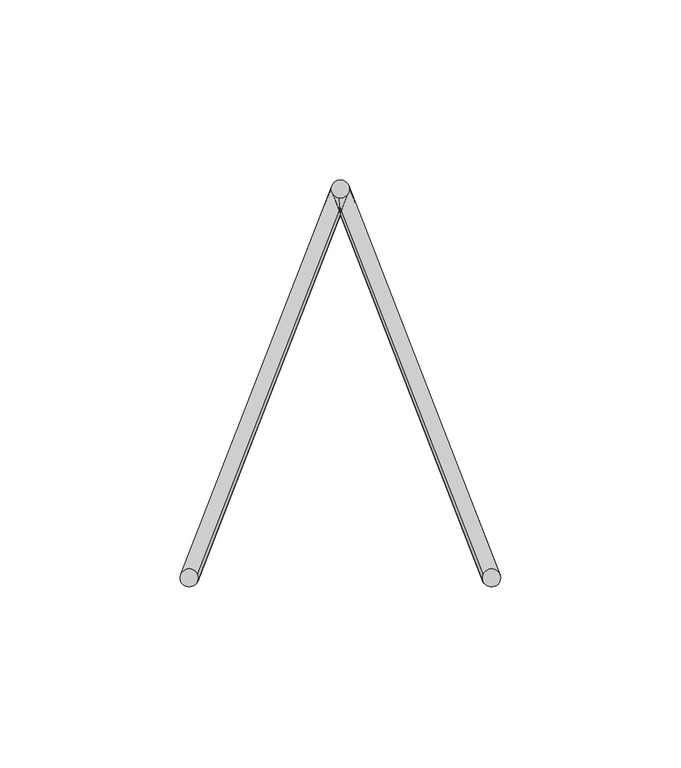
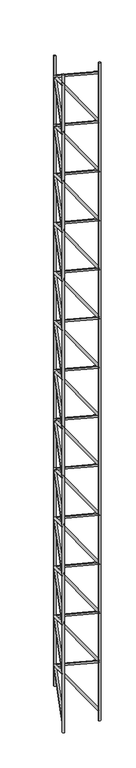
"""IFC4 building model written with IfcOpenShell, lengths in millimetres: proxy geometry, Pre-fab. (Vigota 2 - Pano 8)."""

from ifc_helpers import new_model, si_unit, point, frame, frame_2d, origin, origin_with_axes, origin_2d, place, context, project, spatial, circle_curve, trimmed, segment, composite_curve, outline, extrude, source, transform, mapped, element, save


def structural_framing_c6495f8e(model_context):
    return source(origin(), model_context, "Body", "SweptSolid", [
        extrude(outline(composite_curve([segment(trimmed(circle_curve(origin_2d(), 2.5), [point((2.5, 0.0))], [point((-2.5, 0.0))], False, "CARTESIAN"), True, "CONTINUOUS"), segment(trimmed(circle_curve(origin_2d(), 2.5), [point((-2.5, 0.0))], [point((2.5, 0.0))], False, "CARTESIAN"), True, "CONTINUOUS")], self_intersect=False)), origin_with_axes(), (0.0, 0.0, 1.0), 1607.655183),
        extrude(outline(composite_curve([segment(trimmed(circle_curve(frame_2d((-42.0, 108.0)), 2.5), [point((-39.5, 108.0))], [point((-44.5, 108.0))], False, "CARTESIAN"), True, "CONTINUOUS"), segment(trimmed(circle_curve(frame_2d((-42.0, 108.0)), 2.5), [point((-44.5, 108.0))], [point((-39.5, 108.0))], False, "CARTESIAN"), True, "CONTINUOUS")], self_intersect=False)), frame((0.0, 0.0, 33.8275917), z_axis=(0.0, 0.0, 1.0), x_axis=(1.0, 0.0, 0.0)), (0.0, 0.0, 1.0), 1540.0),
        extrude(outline(composite_curve([segment(trimmed(circle_curve(origin_2d(), 2.5), [point((2.5, 0.0))], [point((-2.5, 0.0))], False, "CARTESIAN"), True, "CONTINUOUS"), segment(trimmed(circle_curve(origin_2d(), 2.5), [point((-2.5, 0.0))], [point((2.5, 0.0))], False, "CARTESIAN"), True, "CONTINUOUS")], self_intersect=False)), frame((0.0, 0.0, 23.8275917), z_axis=(-0.3218603428886276, 0.8276408817707567, 0.4598004898837537), x_axis=(0.8192319205108605, -3.936835275445103e-11, 0.5734623443750141)), (0.0, 0.0, 1.0), 130.491379),
        extrude(outline(composite_curve([segment(trimmed(circle_curve(origin_2d(), 2.5), [point((2.5, 0.0))], [point((-2.5, 0.0))], False, "CARTESIAN"), True, "CONTINUOUS"), segment(trimmed(circle_curve(origin_2d(), 2.5), [point((-2.5, 0.0))], [point((2.5, 0.0))], False, "CARTESIAN"), True, "CONTINUOUS")], self_intersect=False)), frame((-42.0, 108.0, 83.8275917), z_axis=(0.3218603428886276, -0.8276408817707567, 0.4598004898837537), x_axis=(0.8192319205108605, -3.936835275445103e-11, -0.5734623443750141)), (0.0, 0.0, 1.0), 130.491379),
        extrude(outline(composite_curve([segment(trimmed(circle_curve(origin_2d(), 2.5), [point((2.5, 0.0))], [point((-2.5, 0.0))], False, "CARTESIAN"), True, "CONTINUOUS"), segment(trimmed(circle_curve(origin_2d(), 2.5), [point((-2.5, 0.0))], [point((2.5, 0.0))], False, "CARTESIAN"), True, "CONTINUOUS")], self_intersect=False)), frame((0.0, 0.0, 143.8275917), z_axis=(-0.3218603428886276, 0.8276408817707567, 0.4598004898837537), x_axis=(0.8192319205108605, -3.936835275445103e-11, 0.5734623443750141)), (0.0, 0.0, 1.0), 130.491379),
        extrude(outline(composite_curve([segment(trimmed(circle_curve(origin_2d(), 2.5), [point((2.5, 0.0))], [point((-2.5, 0.0))], False, "CARTESIAN"), True, "CONTINUOUS"), segment(trimmed(circle_curve(origin_2d(), 2.5), [point((-2.5, 0.0))], [point((2.5, 0.0))], False, "CARTESIAN"), True, "CONTINUOUS")], self_intersect=False)), frame((-42.0, 108.0, 203.8275917), z_axis=(0.3218603428886276, -0.8276408817707567, 0.4598004898837537), x_axis=(0.8192319205108605, -3.936835275445103e-11, -0.5734623443750141)), (0.0, 0.0, 1.0), 130.491379),
        extrude(outline(composite_curve([segment(trimmed(circle_curve(origin_2d(), 2.5), [point((2.5, 0.0))], [point((-2.5, 0.0))], False, "CARTESIAN"), True, "CONTINUOUS"), segment(trimmed(circle_curve(origin_2d(), 2.5), [point((-2.5, 0.0))], [point((2.5, 0.0))], False, "CARTESIAN"), True, "CONTINUOUS")], self_intersect=False)), frame((0.0, 0.0, 263.8275917), z_axis=(-0.3218603428886276, 0.8276408817707567, 0.4598004898837537), x_axis=(0.8192319205108605, -3.936835275445103e-11, 0.5734623443750141)), (0.0, 0.0, 1.0), 130.491379),
        extrude(outline(composite_curve([segment(trimmed(circle_curve(origin_2d(), 2.5), [point((2.5, 0.0))], [point((-2.5, 0.0))], False, "CARTESIAN"), True, "CONTINUOUS"), segment(trimmed(circle_curve(origin_2d(), 2.5), [point((-2.5, 0.0))], [point((2.5, 0.0))], False, "CARTESIAN"), True, "CONTINUOUS")], self_intersect=False)), frame((-42.0, 108.0, 323.8275917), z_axis=(0.3218603428886276, -0.8276408817707567, 0.4598004898837537), x_axis=(0.8192319205108605, -3.936835275445103e-11, -0.5734623443750141)), (0.0, 0.0, 1.0), 130.491379),
        extrude(outline(composite_curve([segment(trimmed(circle_curve(origin_2d(), 2.5), [point((2.5, 0.0))], [point((-2.5, 0.0))], False, "CARTESIAN"), True, "CONTINUOUS"), segment(trimmed(circle_curve(origin_2d(), 2.5), [point((-2.5, 0.0))], [point((2.5, 0.0))], False, "CARTESIAN"), True, "CONTINUOUS")], self_intersect=False)), frame((0.0, 0.0, 383.8275917), z_axis=(-0.3218603428886276, 0.8276408817707567, 0.4598004898837537), x_axis=(0.8192319205108605, -3.936835275445103e-11, 0.5734623443750141)), (0.0, 0.0, 1.0), 130.491379),
        extrude(outline(composite_curve([segment(trimmed(circle_curve(origin_2d(), 2.5), [point((2.5, 0.0))], [point((-2.5, 0.0))], False, "CARTESIAN"), True, "CONTINUOUS"), segment(trimmed(circle_curve(origin_2d(), 2.5), [point((-2.5, 0.0))], [point((2.5, 0.0))], False, "CARTESIAN"), True, "CONTINUOUS")], self_intersect=False)), frame((-42.0, 108.0, 443.8275917), z_axis=(0.3218603428886276, -0.8276408817707567, 0.4598004898837537), x_axis=(0.8192319205108605, -3.936835275445103e-11, -0.5734623443750141)), (0.0, 0.0, 1.0), 130.491379),
        extrude(outline(composite_curve([segment(trimmed(circle_curve(origin_2d(), 2.5), [point((2.5, 0.0))], [point((-2.5, 0.0))], False, "CARTESIAN"), True, "CONTINUOUS"), segment(trimmed(circle_curve(origin_2d(), 2.5), [point((-2.5, 0.0))], [point((2.5, 0.0))], False, "CARTESIAN"), True, "CONTINUOUS")], self_intersect=False)), frame((0.0, 0.0, 503.8275917), z_axis=(-0.3218603428886276, 0.8276408817707567, 0.4598004898837537), x_axis=(0.8192319205108605, -3.936835275445103e-11, 0.5734623443750141)), (0.0, 0.0, 1.0), 130.491379),
        extrude(outline(composite_curve([segment(trimmed(circle_curve(origin_2d(), 2.5), [point((2.5, 0.0))], [point((-2.5, 0.0))], False, "CARTESIAN"), True, "CONTINUOUS"), segment(trimmed(circle_curve(origin_2d(), 2.5), [point((-2.5, 0.0))], [point((2.5, 0.0))], False, "CARTESIAN"), True, "CONTINUOUS")], self_intersect=False)), frame((-42.0, 108.0, 563.8275917), z_axis=(0.3218603428886276, -0.8276408817707567, 0.4598004898837537), x_axis=(0.8192319205108605, -3.936835275445103e-11, -0.5734623443750141)), (0.0, 0.0, 1.0), 130.491379),
        extrude(outline(composite_curve([segment(trimmed(circle_curve(origin_2d(), 2.5), [point((2.5, 0.0))], [point((-2.5, 0.0))], False, "CARTESIAN"), True, "CONTINUOUS"), segment(trimmed(circle_curve(origin_2d(), 2.5), [point((-2.5, 0.0))], [point((2.5, 0.0))], False, "CARTESIAN"), True, "CONTINUOUS")], self_intersect=False)), frame((0.0, 0.0, 623.8275917), z_axis=(-0.3218603428886276, 0.8276408817707567, 0.4598004898837537), x_axis=(0.8192319205108605, -3.936835275445103e-11, 0.5734623443750141)), (0.0, 0.0, 1.0), 130.491379),
        extrude(outline(composite_curve([segment(trimmed(circle_curve(origin_2d(), 2.5), [point((2.5, 0.0))], [point((-2.5, 0.0))], False, "CARTESIAN"), True, "CONTINUOUS"), segment(trimmed(circle_curve(origin_2d(), 2.5), [point((-2.5, 0.0))], [point((2.5, 0.0))], False, "CARTESIAN"), True, "CONTINUOUS")], self_intersect=False)), frame((-42.0, 108.0, 683.8275917), z_axis=(0.3218603428886276, -0.8276408817707567, 0.4598004898837537), x_axis=(0.8192319205108605, -3.936835275445103e-11, -0.5734623443750141)), (0.0, 0.0, 1.0), 130.491379),
        extrude(outline(composite_curve([segment(trimmed(circle_curve(origin_2d(), 2.5), [point((2.5, 0.0))], [point((-2.5, 0.0))], False, "CARTESIAN"), True, "CONTINUOUS"), segment(trimmed(circle_curve(origin_2d(), 2.5), [point((-2.5, 0.0))], [point((2.5, 0.0))], False, "CARTESIAN"), True, "CONTINUOUS")], self_intersect=False)), frame((0.0, 0.0, 743.8275917), z_axis=(-0.3218603428886276, 0.8276408817707567, 0.4598004898837537), x_axis=(0.8192319205108605, -3.936835275445103e-11, 0.5734623443750141)), (0.0, 0.0, 1.0), 130.491379),
        extrude(outline(composite_curve([segment(trimmed(circle_curve(origin_2d(), 2.5), [point((2.5, 0.0))], [point((-2.5, 0.0))], False, "CARTESIAN"), True, "CONTINUOUS"), segment(trimmed(circle_curve(origin_2d(), 2.5), [point((-2.5, 0.0))], [point((2.5, 0.0))], False, "CARTESIAN"), True, "CONTINUOUS")], self_intersect=False)), frame((-42.0, 108.0, 803.8275917), z_axis=(0.3218603428886276, -0.8276408817707567, 0.4598004898837537), x_axis=(0.8192319205108605, -3.936835275445103e-11, -0.5734623443750141)), (0.0, 0.0, 1.0), 130.491379),
        extrude(outline(composite_curve([segment(trimmed(circle_curve(origin_2d(), 2.5), [point((2.5, 0.0))], [point((-2.5, 0.0))], False, "CARTESIAN"), True, "CONTINUOUS"), segment(trimmed(circle_curve(origin_2d(), 2.5), [point((-2.5, 0.0))], [point((2.5, 0.0))], False, "CARTESIAN"), True, "CONTINUOUS")], self_intersect=False)), frame((0.0, 0.0, 863.8275917), z_axis=(-0.3218603428886276, 0.8276408817707567, 0.4598004898837537), x_axis=(0.8192319205108605, -3.936835275445103e-11, 0.5734623443750141)), (0.0, 0.0, 1.0), 130.491379),
        extrude(outline(composite_curve([segment(trimmed(circle_curve(origin_2d(), 2.5), [point((2.5, 0.0))], [point((-2.5, 0.0))], False, "CARTESIAN"), True, "CONTINUOUS"), segment(trimmed(circle_curve(origin_2d(), 2.5), [point((-2.5, 0.0))], [point((2.5, 0.0))], False, "CARTESIAN"), True, "CONTINUOUS")], self_intersect=False)), frame((-42.0, 108.0, 923.8275917), z_axis=(0.3218603428886276, -0.8276408817707567, 0.4598004898837537), x_axis=(0.8192319205108605, -3.936835275445103e-11, -0.5734623443750141)), (0.0, 0.0, 1.0), 130.491379),
        extrude(outline(composite_curve([segment(trimmed(circle_curve(origin_2d(), 2.5), [point((2.5, 0.0))], [point((-2.5, 0.0))], False, "CARTESIAN"), True, "CONTINUOUS"), segment(trimmed(circle_curve(origin_2d(), 2.5), [point((-2.5, 0.0))], [point((2.5, 0.0))], False, "CARTESIAN"), True, "CONTINUOUS")], self_intersect=False)), frame((0.0, 0.0, 983.8275917), z_axis=(-0.3218603428886276, 0.8276408817707567, 0.4598004898837537), x_axis=(0.8192319205108605, -3.936835275445103e-11, 0.5734623443750141)), (0.0, 0.0, 1.0), 130.491379),
        extrude(outline(composite_curve([segment(trimmed(circle_curve(origin_2d(), 2.5), [point((2.5, 0.0))], [point((-2.5, 0.0))], False, "CARTESIAN"), True, "CONTINUOUS"), segment(trimmed(circle_curve(origin_2d(), 2.5), [point((-2.5, 0.0))], [point((2.5, 0.0))], False, "CARTESIAN"), True, "CONTINUOUS")], self_intersect=False)), frame((-42.0, 108.0, 1043.827592), z_axis=(0.3218603428886276, -0.8276408817707567, 0.4598004898837537), x_axis=(0.8192319205108605, -3.936835275445103e-11, -0.5734623443750141)), (0.0, 0.0, 1.0), 130.491379),
        extrude(outline(composite_curve([segment(trimmed(circle_curve(origin_2d(), 2.5), [point((2.5, 0.0))], [point((-2.5, 0.0))], False, "CARTESIAN"), True, "CONTINUOUS"), segment(trimmed(circle_curve(origin_2d(), 2.5), [point((-2.5, 0.0))], [point((2.5, 0.0))], False, "CARTESIAN"), True, "CONTINUOUS")], self_intersect=False)), frame((0.0, 0.0, 1103.827592), z_axis=(-0.3218603428886276, 0.8276408817707567, 0.4598004898837537), x_axis=(0.8192319205108605, -3.936835275445103e-11, 0.5734623443750141)), (0.0, 0.0, 1.0), 130.491379),
        extrude(outline(composite_curve([segment(trimmed(circle_curve(origin_2d(), 2.5), [point((2.5, 0.0))], [point((-2.5, 0.0))], False, "CARTESIAN"), True, "CONTINUOUS"), segment(trimmed(circle_curve(origin_2d(), 2.5), [point((-2.5, 0.0))], [point((2.5, 0.0))], False, "CARTESIAN"), True, "CONTINUOUS")], self_intersect=False)), frame((-42.0, 108.0, 1163.827592), z_axis=(0.3218603428886276, -0.8276408817707567, 0.4598004898837537), x_axis=(0.8192319205108605, -3.936835275445103e-11, -0.5734623443750141)), (0.0, 0.0, 1.0), 130.491379),
        extrude(outline(composite_curve([segment(trimmed(circle_curve(origin_2d(), 2.5), [point((2.5, 0.0))], [point((-2.5, 0.0))], False, "CARTESIAN"), True, "CONTINUOUS"), segment(trimmed(circle_curve(origin_2d(), 2.5), [point((-2.5, 0.0))], [point((2.5, 0.0))], False, "CARTESIAN"), True, "CONTINUOUS")], self_intersect=False)), frame((0.0, 0.0, 1223.827592), z_axis=(-0.3218603428886276, 0.8276408817707567, 0.4598004898837537), x_axis=(0.8192319205108605, -3.936835275445103e-11, 0.5734623443750141)), (0.0, 0.0, 1.0), 130.491379),
        extrude(outline(composite_curve([segment(trimmed(circle_curve(origin_2d(), 2.5), [point((2.5, 0.0))], [point((-2.5, 0.0))], False, "CARTESIAN"), True, "CONTINUOUS"), segment(trimmed(circle_curve(origin_2d(), 2.5), [point((-2.5, 0.0))], [point((2.5, 0.0))], False, "CARTESIAN"), True, "CONTINUOUS")], self_intersect=False)), frame((-42.0, 108.0, 1283.827592), z_axis=(0.3218603428886276, -0.8276408817707567, 0.4598004898837537), x_axis=(0.8192319205108605, -3.936835275445103e-11, -0.5734623443750141)), (0.0, 0.0, 1.0), 130.491379),
        extrude(outline(composite_curve([segment(trimmed(circle_curve(origin_2d(), 2.5), [point((2.5, 0.0))], [point((-2.5, 0.0))], False, "CARTESIAN"), True, "CONTINUOUS"), segment(trimmed(circle_curve(origin_2d(), 2.5), [point((-2.5, 0.0))], [point((2.5, 0.0))], False, "CARTESIAN"), True, "CONTINUOUS")], self_intersect=False)), frame((0.0, 0.0, 1343.827592), z_axis=(-0.3218603428886276, 0.8276408817707567, 0.4598004898837537), x_axis=(0.8192319205108605, -3.936835275445103e-11, 0.5734623443750141)), (0.0, 0.0, 1.0), 130.491379),
        extrude(outline(composite_curve([segment(trimmed(circle_curve(origin_2d(), 2.5), [point((2.5, 0.0))], [point((-2.5, 0.0))], False, "CARTESIAN"), True, "CONTINUOUS"), segment(trimmed(circle_curve(origin_2d(), 2.5), [point((-2.5, 0.0))], [point((2.5, 0.0))], False, "CARTESIAN"), True, "CONTINUOUS")], self_intersect=False)), frame((-42.0, 108.0, 1403.827592), z_axis=(0.3218603428886276, -0.8276408817707567, 0.4598004898837537), x_axis=(0.8192319205108605, -3.936835275445103e-11, -0.5734623443750141)), (0.0, 0.0, 1.0), 130.491379),
        extrude(outline(composite_curve([segment(trimmed(circle_curve(origin_2d(), 2.5), [point((2.5, 0.0))], [point((-2.5, 0.0))], False, "CARTESIAN"), True, "CONTINUOUS"), segment(trimmed(circle_curve(origin_2d(), 2.5), [point((-2.5, 0.0))], [point((2.5, 0.0))], False, "CARTESIAN"), True, "CONTINUOUS")], self_intersect=False)), frame((0.0, 0.0, 1463.827592), z_axis=(-0.3218603428886276, 0.8276408817707567, 0.4598004898837537), x_axis=(0.8192319205108605, -3.936835275445103e-11, 0.5734623443750141)), (0.0, 0.0, 1.0), 130.491379),
        extrude(outline(composite_curve([segment(trimmed(circle_curve(origin_2d(), 2.5), [point((2.5, 0.0))], [point((-2.5, 0.0))], False, "CARTESIAN"), True, "CONTINUOUS"), segment(trimmed(circle_curve(origin_2d(), 2.5), [point((-2.5, 0.0))], [point((2.5, 0.0))], False, "CARTESIAN"), True, "CONTINUOUS")], self_intersect=False)), frame((-42.0, 108.0, 1523.827592), z_axis=(0.3218603428886276, -0.8276408817707567, 0.4598004898837537), x_axis=(0.8192319205108605, -3.936835275445103e-11, -0.5734623443750141)), (0.0, 0.0, 1.0), 130.491379),
        extrude(outline(composite_curve([segment(trimmed(circle_curve(frame_2d((-84.0, 0.0)), 2.5), [point((-81.5, 0.0))], [point((-86.5, 0.0))], False, "CARTESIAN"), True, "CONTINUOUS"), segment(trimmed(circle_curve(frame_2d((-84.0, 0.0)), 2.5), [point((-86.5, 0.0))], [point((-81.5, 0.0))], False, "CARTESIAN"), True, "CONTINUOUS")], self_intersect=False)), origin_with_axes(), (0.0, 0.0, 1.0), 1607.655183),
        extrude(outline(composite_curve([segment(trimmed(circle_curve(origin_2d(), 2.5), [point((2.5, 0.0))], [point((-2.5, 0.0))], False, "CARTESIAN"), True, "CONTINUOUS"), segment(trimmed(circle_curve(origin_2d(), 2.5), [point((-2.5, 0.0))], [point((2.5, 0.0))], False, "CARTESIAN"), True, "CONTINUOUS")], self_intersect=False)), frame((-84.0, 0.0, 23.8275917), z_axis=(0.3218603428886276, 0.8276408817707567, 0.4598004898837537), x_axis=(0.8192319205108605, 3.936835275445103e-11, -0.5734623443750141)), (0.0, 0.0, 1.0), 130.491379),
        extrude(outline(composite_curve([segment(trimmed(circle_curve(origin_2d(), 2.5), [point((2.5, 0.0))], [point((-2.5, 0.0))], False, "CARTESIAN"), True, "CONTINUOUS"), segment(trimmed(circle_curve(origin_2d(), 2.5), [point((-2.5, 0.0))], [point((2.5, 0.0))], False, "CARTESIAN"), True, "CONTINUOUS")], self_intersect=False)), frame((-42.0, 108.0, 83.8275917), z_axis=(-0.3218603428886276, -0.8276408817707567, 0.4598004898837537), x_axis=(0.8192319205108605, 3.936835275445103e-11, 0.5734623443750141)), (0.0, 0.0, 1.0), 130.491379),
        extrude(outline(composite_curve([segment(trimmed(circle_curve(origin_2d(), 2.5), [point((2.5, 0.0))], [point((-2.5, 0.0))], False, "CARTESIAN"), True, "CONTINUOUS"), segment(trimmed(circle_curve(origin_2d(), 2.5), [point((-2.5, 0.0))], [point((2.5, 0.0))], False, "CARTESIAN"), True, "CONTINUOUS")], self_intersect=False)), frame((-84.0, 0.0, 143.8275917), z_axis=(0.3218603428886276, 0.8276408817707567, 0.4598004898837537), x_axis=(0.8192319205108605, 3.936835275445103e-11, -0.5734623443750141)), (0.0, 0.0, 1.0), 130.491379),
        extrude(outline(composite_curve([segment(trimmed(circle_curve(origin_2d(), 2.5), [point((2.5, 0.0))], [point((-2.5, 0.0))], False, "CARTESIAN"), True, "CONTINUOUS"), segment(trimmed(circle_curve(origin_2d(), 2.5), [point((-2.5, 0.0))], [point((2.5, 0.0))], False, "CARTESIAN"), True, "CONTINUOUS")], self_intersect=False)), frame((-42.0, 108.0, 203.8275917), z_axis=(-0.3218603428886276, -0.8276408817707567, 0.4598004898837537), x_axis=(0.8192319205108605, 3.936835275445103e-11, 0.5734623443750141)), (0.0, 0.0, 1.0), 130.491379),
        extrude(outline(composite_curve([segment(trimmed(circle_curve(origin_2d(), 2.5), [point((2.5, 0.0))], [point((-2.5, 0.0))], False, "CARTESIAN"), True, "CONTINUOUS"), segment(trimmed(circle_curve(origin_2d(), 2.5), [point((-2.5, 0.0))], [point((2.5, 0.0))], False, "CARTESIAN"), True, "CONTINUOUS")], self_intersect=False)), frame((-84.0, 0.0, 263.8275917), z_axis=(0.3218603428886276, 0.8276408817707567, 0.4598004898837537), x_axis=(0.8192319205108605, 3.936835275445103e-11, -0.5734623443750141)), (0.0, 0.0, 1.0), 130.491379),
        extrude(outline(composite_curve([segment(trimmed(circle_curve(origin_2d(), 2.5), [point((2.5, 0.0))], [point((-2.5, 0.0))], False, "CARTESIAN"), True, "CONTINUOUS"), segment(trimmed(circle_curve(origin_2d(), 2.5), [point((-2.5, 0.0))], [point((2.5, 0.0))], False, "CARTESIAN"), True, "CONTINUOUS")], self_intersect=False)), frame((-42.0, 108.0, 323.8275917), z_axis=(-0.3218603428886276, -0.8276408817707567, 0.4598004898837537), x_axis=(0.8192319205108605, 3.936835275445103e-11, 0.5734623443750141)), (0.0, 0.0, 1.0), 130.491379),
        extrude(outline(composite_curve([segment(trimmed(circle_curve(origin_2d(), 2.5), [point((2.5, 0.0))], [point((-2.5, 0.0))], False, "CARTESIAN"), True, "CONTINUOUS"), segment(trimmed(circle_curve(origin_2d(), 2.5), [point((-2.5, 0.0))], [point((2.5, 0.0))], False, "CARTESIAN"), True, "CONTINUOUS")], self_intersect=False)), frame((-84.0, 0.0, 383.8275917), z_axis=(0.3218603428886276, 0.8276408817707567, 0.4598004898837537), x_axis=(0.8192319205108605, 3.936835275445103e-11, -0.5734623443750141)), (0.0, 0.0, 1.0), 130.491379),
        extrude(outline(composite_curve([segment(trimmed(circle_curve(origin_2d(), 2.5), [point((2.5, 0.0))], [point((-2.5, 0.0))], False, "CARTESIAN"), True, "CONTINUOUS"), segment(trimmed(circle_curve(origin_2d(), 2.5), [point((-2.5, 0.0))], [point((2.5, 0.0))], False, "CARTESIAN"), True, "CONTINUOUS")], self_intersect=False)), frame((-42.0, 108.0, 443.8275917), z_axis=(-0.3218603428886276, -0.8276408817707567, 0.4598004898837537), x_axis=(0.8192319205108605, 3.936835275445103e-11, 0.5734623443750141)), (0.0, 0.0, 1.0), 130.491379),
        extrude(outline(composite_curve([segment(trimmed(circle_curve(origin_2d(), 2.5), [point((2.5, 0.0))], [point((-2.5, 0.0))], False, "CARTESIAN"), True, "CONTINUOUS"), segment(trimmed(circle_curve(origin_2d(), 2.5), [point((-2.5, 0.0))], [point((2.5, 0.0))], False, "CARTESIAN"), True, "CONTINUOUS")], self_intersect=False)), frame((-84.0, 0.0, 503.8275917), z_axis=(0.3218603428886276, 0.8276408817707567, 0.4598004898837537), x_axis=(0.8192319205108605, 3.936835275445103e-11, -0.5734623443750141)), (0.0, 0.0, 1.0), 130.491379),
        extrude(outline(composite_curve([segment(trimmed(circle_curve(origin_2d(), 2.5), [point((2.5, 0.0))], [point((-2.5, 0.0))], False, "CARTESIAN"), True, "CONTINUOUS"), segment(trimmed(circle_curve(origin_2d(), 2.5), [point((-2.5, 0.0))], [point((2.5, 0.0))], False, "CARTESIAN"), True, "CONTINUOUS")], self_intersect=False)), frame((-42.0, 108.0, 563.8275917), z_axis=(-0.3218603428886276, -0.8276408817707567, 0.4598004898837537), x_axis=(0.8192319205108605, 3.936835275445103e-11, 0.5734623443750141)), (0.0, 0.0, 1.0), 130.491379),
        extrude(outline(composite_curve([segment(trimmed(circle_curve(origin_2d(), 2.5), [point((2.5, 0.0))], [point((-2.5, 0.0))], False, "CARTESIAN"), True, "CONTINUOUS"), segment(trimmed(circle_curve(origin_2d(), 2.5), [point((-2.5, 0.0))], [point((2.5, 0.0))], False, "CARTESIAN"), True, "CONTINUOUS")], self_intersect=False)), frame((-84.0, 0.0, 623.8275917), z_axis=(0.3218603428886276, 0.8276408817707567, 0.4598004898837537), x_axis=(0.8192319205108605, 3.936835275445103e-11, -0.5734623443750141)), (0.0, 0.0, 1.0), 130.491379),
        extrude(outline(composite_curve([segment(trimmed(circle_curve(origin_2d(), 2.5), [point((2.5, 0.0))], [point((-2.5, 0.0))], False, "CARTESIAN"), True, "CONTINUOUS"), segment(trimmed(circle_curve(origin_2d(), 2.5), [point((-2.5, 0.0))], [point((2.5, 0.0))], False, "CARTESIAN"), True, "CONTINUOUS")], self_intersect=False)), frame((-42.0, 108.0, 683.8275917), z_axis=(-0.3218603428886276, -0.8276408817707567, 0.4598004898837537), x_axis=(0.8192319205108605, 3.936835275445103e-11, 0.5734623443750141)), (0.0, 0.0, 1.0), 130.491379),
        extrude(outline(composite_curve([segment(trimmed(circle_curve(origin_2d(), 2.5), [point((2.5, 0.0))], [point((-2.5, 0.0))], False, "CARTESIAN"), True, "CONTINUOUS"), segment(trimmed(circle_curve(origin_2d(), 2.5), [point((-2.5, 0.0))], [point((2.5, 0.0))], False, "CARTESIAN"), True, "CONTINUOUS")], self_intersect=False)), frame((-84.0, 0.0, 743.8275917), z_axis=(0.3218603428886276, 0.8276408817707567, 0.4598004898837537), x_axis=(0.8192319205108605, 3.936835275445103e-11, -0.5734623443750141)), (0.0, 0.0, 1.0), 130.491379),
        extrude(outline(composite_curve([segment(trimmed(circle_curve(origin_2d(), 2.5), [point((2.5, 0.0))], [point((-2.5, 0.0))], False, "CARTESIAN"), True, "CONTINUOUS"), segment(trimmed(circle_curve(origin_2d(), 2.5), [point((-2.5, 0.0))], [point((2.5, 0.0))], False, "CARTESIAN"), True, "CONTINUOUS")], self_intersect=False)), frame((-42.0, 108.0, 803.8275917), z_axis=(-0.3218603428886276, -0.8276408817707567, 0.4598004898837537), x_axis=(0.8192319205108605, 3.936835275445103e-11, 0.5734623443750141)), (0.0, 0.0, 1.0), 130.491379),
        extrude(outline(composite_curve([segment(trimmed(circle_curve(origin_2d(), 2.5), [point((2.5, 0.0))], [point((-2.5, 0.0))], False, "CARTESIAN"), True, "CONTINUOUS"), segment(trimmed(circle_curve(origin_2d(), 2.5), [point((-2.5, 0.0))], [point((2.5, 0.0))], False, "CARTESIAN"), True, "CONTINUOUS")], self_intersect=False)), frame((-84.0, 0.0, 863.8275917), z_axis=(0.3218603428886276, 0.8276408817707567, 0.4598004898837537), x_axis=(0.8192319205108605, 3.936835275445103e-11, -0.5734623443750141)), (0.0, 0.0, 1.0), 130.491379),
        extrude(outline(composite_curve([segment(trimmed(circle_curve(origin_2d(), 2.5), [point((2.5, 0.0))], [point((-2.5, 0.0))], False, "CARTESIAN"), True, "CONTINUOUS"), segment(trimmed(circle_curve(origin_2d(), 2.5), [point((-2.5, 0.0))], [point((2.5, 0.0))], False, "CARTESIAN"), True, "CONTINUOUS")], self_intersect=False)), frame((-42.0, 108.0, 923.8275917), z_axis=(-0.3218603428886276, -0.8276408817707567, 0.4598004898837537), x_axis=(0.8192319205108605, 3.936835275445103e-11, 0.5734623443750141)), (0.0, 0.0, 1.0), 130.491379),
        extrude(outline(composite_curve([segment(trimmed(circle_curve(origin_2d(), 2.5), [point((2.5, 0.0))], [point((-2.5, 0.0))], False, "CARTESIAN"), True, "CONTINUOUS"), segment(trimmed(circle_curve(origin_2d(), 2.5), [point((-2.5, 0.0))], [point((2.5, 0.0))], False, "CARTESIAN"), True, "CONTINUOUS")], self_intersect=False)), frame((-84.0, 0.0, 983.8275917), z_axis=(0.3218603428886276, 0.8276408817707567, 0.4598004898837537), x_axis=(0.8192319205108605, 3.936835275445103e-11, -0.5734623443750141)), (0.0, 0.0, 1.0), 130.491379),
        extrude(outline(composite_curve([segment(trimmed(circle_curve(origin_2d(), 2.5), [point((2.5, 0.0))], [point((-2.5, 0.0))], False, "CARTESIAN"), True, "CONTINUOUS"), segment(trimmed(circle_curve(origin_2d(), 2.5), [point((-2.5, 0.0))], [point((2.5, 0.0))], False, "CARTESIAN"), True, "CONTINUOUS")], self_intersect=False)), frame((-42.0, 108.0, 1043.827592), z_axis=(-0.3218603428886276, -0.8276408817707567, 0.4598004898837537), x_axis=(0.8192319205108605, 3.936835275445103e-11, 0.5734623443750141)), (0.0, 0.0, 1.0), 130.491379),
        extrude(outline(composite_curve([segment(trimmed(circle_curve(origin_2d(), 2.5), [point((2.5, 0.0))], [point((-2.5, 0.0))], False, "CARTESIAN"), True, "CONTINUOUS"), segment(trimmed(circle_curve(origin_2d(), 2.5), [point((-2.5, 0.0))], [point((2.5, 0.0))], False, "CARTESIAN"), True, "CONTINUOUS")], self_intersect=False)), frame((-84.0, 0.0, 1103.827592), z_axis=(0.3218603428886276, 0.8276408817707567, 0.4598004898837537), x_axis=(0.8192319205108605, 3.936835275445103e-11, -0.5734623443750141)), (0.0, 0.0, 1.0), 130.491379),
        extrude(outline(composite_curve([segment(trimmed(circle_curve(origin_2d(), 2.5), [point((2.5, 0.0))], [point((-2.5, 0.0))], False, "CARTESIAN"), True, "CONTINUOUS"), segment(trimmed(circle_curve(origin_2d(), 2.5), [point((-2.5, 0.0))], [point((2.5, 0.0))], False, "CARTESIAN"), True, "CONTINUOUS")], self_intersect=False)), frame((-42.0, 108.0, 1163.827592), z_axis=(-0.3218603428886276, -0.8276408817707567, 0.4598004898837537), x_axis=(0.8192319205108605, 3.936835275445103e-11, 0.5734623443750141)), (0.0, 0.0, 1.0), 130.491379),
        extrude(outline(composite_curve([segment(trimmed(circle_curve(origin_2d(), 2.5), [point((2.5, 0.0))], [point((-2.5, 0.0))], False, "CARTESIAN"), True, "CONTINUOUS"), segment(trimmed(circle_curve(origin_2d(), 2.5), [point((-2.5, 0.0))], [point((2.5, 0.0))], False, "CARTESIAN"), True, "CONTINUOUS")], self_intersect=False)), frame((-84.0, 0.0, 1223.827592), z_axis=(0.3218603428886276, 0.8276408817707567, 0.4598004898837537), x_axis=(0.8192319205108605, 3.936835275445103e-11, -0.5734623443750141)), (0.0, 0.0, 1.0), 130.491379),
        extrude(outline(composite_curve([segment(trimmed(circle_curve(origin_2d(), 2.5), [point((2.5, 0.0))], [point((-2.5, 0.0))], False, "CARTESIAN"), True, "CONTINUOUS"), segment(trimmed(circle_curve(origin_2d(), 2.5), [point((-2.5, 0.0))], [point((2.5, 0.0))], False, "CARTESIAN"), True, "CONTINUOUS")], self_intersect=False)), frame((-42.0, 108.0, 1283.827592), z_axis=(-0.3218603428886276, -0.8276408817707567, 0.4598004898837537), x_axis=(0.8192319205108605, 3.936835275445103e-11, 0.5734623443750141)), (0.0, 0.0, 1.0), 130.491379),
        extrude(outline(composite_curve([segment(trimmed(circle_curve(origin_2d(), 2.5), [point((2.5, 0.0))], [point((-2.5, 0.0))], False, "CARTESIAN"), True, "CONTINUOUS"), segment(trimmed(circle_curve(origin_2d(), 2.5), [point((-2.5, 0.0))], [point((2.5, 0.0))], False, "CARTESIAN"), True, "CONTINUOUS")], self_intersect=False)), frame((-84.0, 0.0, 1343.827592), z_axis=(0.3218603428886276, 0.8276408817707567, 0.4598004898837537), x_axis=(0.8192319205108605, 3.936835275445103e-11, -0.5734623443750141)), (0.0, 0.0, 1.0), 130.491379),
        extrude(outline(composite_curve([segment(trimmed(circle_curve(origin_2d(), 2.5), [point((2.5, 0.0))], [point((-2.5, 0.0))], False, "CARTESIAN"), True, "CONTINUOUS"), segment(trimmed(circle_curve(origin_2d(), 2.5), [point((-2.5, 0.0))], [point((2.5, 0.0))], False, "CARTESIAN"), True, "CONTINUOUS")], self_intersect=False)), frame((-42.0, 108.0, 1403.827592), z_axis=(-0.3218603428886276, -0.8276408817707567, 0.4598004898837537), x_axis=(0.8192319205108605, 3.936835275445103e-11, 0.5734623443750141)), (0.0, 0.0, 1.0), 130.491379),
        extrude(outline(composite_curve([segment(trimmed(circle_curve(origin_2d(), 2.5), [point((2.5, 0.0))], [point((-2.5, 0.0))], False, "CARTESIAN"), True, "CONTINUOUS"), segment(trimmed(circle_curve(origin_2d(), 2.5), [point((-2.5, 0.0))], [point((2.5, 0.0))], False, "CARTESIAN"), True, "CONTINUOUS")], self_intersect=False)), frame((-84.0, 0.0, 1463.827592), z_axis=(0.3218603428886276, 0.8276408817707567, 0.4598004898837537), x_axis=(0.8192319205108605, 3.936835275445103e-11, -0.5734623443750141)), (0.0, 0.0, 1.0), 130.491379),
        extrude(outline(composite_curve([segment(trimmed(circle_curve(origin_2d(), 2.5), [point((2.5, 0.0))], [point((-2.5, 0.0))], False, "CARTESIAN"), True, "CONTINUOUS"), segment(trimmed(circle_curve(origin_2d(), 2.5), [point((-2.5, 0.0))], [point((2.5, 0.0))], False, "CARTESIAN"), True, "CONTINUOUS")], self_intersect=False)), frame((-42.0, 108.0, 1523.827592), z_axis=(-0.3218603428886276, -0.8276408817707567, 0.4598004898837537), x_axis=(0.8192319205108605, 3.936835275445103e-11, 0.5734623443750141)), (0.0, 0.0, 1.0), 130.491379),
    ])


if __name__ == "__main__":
    model = new_model("IFC4")
    model_context = context("Model", 3, world=origin())
    ifc_project = project(units=[si_unit("LENGTHUNIT", "METRE", prefix="MILLI")], contexts=[model_context])
    site = spatial("IfcSite", under=ifc_project)
    building = spatial("IfcBuilding", under=site)
    placement = place(None, origin())
    structural_framing_shape = structural_framing_c6495f8e(model_context)
    element("IfcBuildingElementProxy", 1, Name="Pre-fab. (Vigota 2 - Pano 8)", ObjectType="Pre-fab. (Vigota 2 - Pano 8)", at=placement, inside=building, context=model_context, shape_type="MappedRepresentation", body=[
        mapped(structural_framing_shape, transform((0.0, 0.0, 0.0), x_axis=(1.0, 0.0, 0.0), y_axis=(0.0, 1.0, 0.0), z_axis=(0.0, 0.0, 1.0))),
    ])
    save(model, "model.ifc")

# Revit data of these elements
# Element 1 (IfcBuildingElementProxy, "Pre-fab. (Vigota 2 - Pano 8)")
#   Materials on its faces: "Aço"
# Materials
#   "Aço": class "Metal", colour RGB 120 120 120, transparency 0, Description = "Aço estrutural A36 grau, ASTM B, acabamento laminado", Cost = 0
